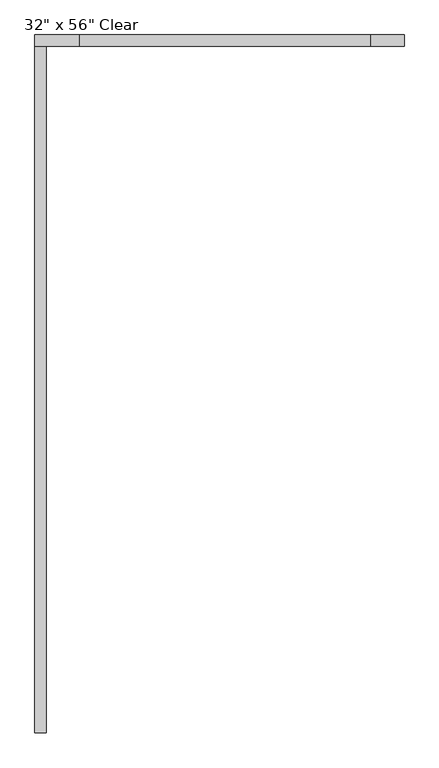
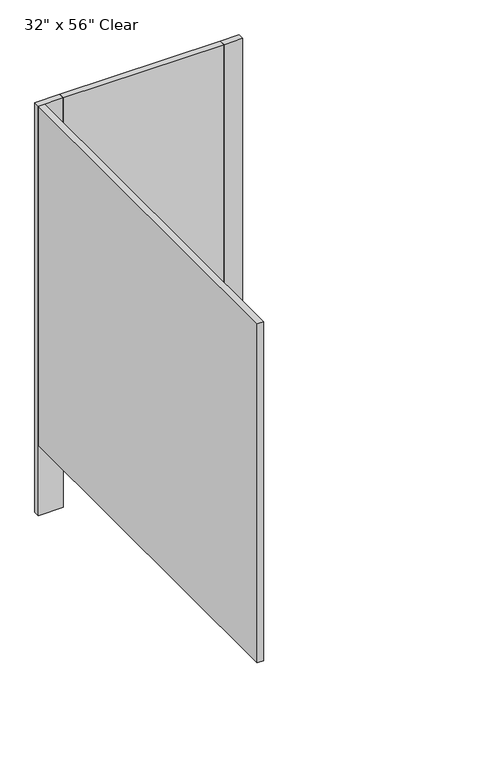
"""IFC4 building model written with IfcOpenShell, lengths in millimetres: proxy geometry."""

from ifc_helpers import new_model, si_unit, frame, origin, origin_with_axes, place, context, project, spatial, polyline, outline, extrude, source, transform, mapped, element, save


def proxy_86d28e76(model_context):
    return source(origin(), model_context, "Body", "SweptSolid", [
        extrude(outline(polyline([(735.1031538, 1646.2375), (735.1031538, 1620.8375), (74.7031538, 1620.8375), (74.7031538, 1646.2375), (735.1031538, 1646.2375)])), frame((0.0, 0.0, 304.8), z_axis=(0.0, 0.0, 1.0), x_axis=(1.0, 0.0, 0.0)), (0.0, 0.0, 1.0), 1473.2),
        extrude(outline(polyline([(74.7031538, 1646.2375), (74.7031538, 1620.8375), (-26.8968462, 1620.8375), (-26.8968462, 1646.2375), (74.7031538, 1646.2375)])), origin_with_axes(), (0.0, 0.0, 1.0), 1778.0),
        extrude(outline(polyline([(811.3031538, 1646.2375), (811.3031538, 1620.8375), (735.1031538, 1620.8375), (735.1031538, 1646.2375), (811.3031538, 1646.2375)])), origin_with_axes(), (0.0, 0.0, 1.0), 1778.0),
        extrude(outline(polyline([(-26.8968462, 1620.8375), (-1.4968462, 1620.8375), (-1.4968462, 63.5), (-26.8968462, 63.5), (-26.8968462, 1620.8375)])), frame((0.0, 0.0, 304.8), z_axis=(0.0, 0.0, 1.0), x_axis=(1.0, 0.0, 0.0)), (0.0, 0.0, 1.0), 1473.2),
    ])


if __name__ == "__main__":
    model = new_model("IFC4")
    model_context = context("Model", 3, world=origin())
    ifc_project = project(units=[si_unit("LENGTHUNIT", "METRE", prefix="MILLI")], contexts=[model_context])
    site = spatial("IfcSite", under=ifc_project)
    building = spatial("IfcBuilding", under=site)
    placement = place(None, origin())
    proxy_shape = proxy_86d28e76(model_context)
    element("IfcBuildingElementProxy", 1, Name="Toilet Stall-3D w Toilet : 32\" x 56\" Clear", ObjectType="Toilet Stall-3D w Toilet : 32\" x 56\" Clear", at=placement, inside=building, context=model_context, shape_type="MappedRepresentation", body=[
        mapped(proxy_shape, transform((0.0, 0.0, 0.0), x_axis=(1.0, 0.0, 0.0), y_axis=(0.0, 1.0, 0.0), z_axis=(0.0, 0.0, 1.0))),
    ])
    save(model, "model.ifc")

# Revit data of these elements
# Type "Toilet Stall-3D w Toilet : 32\" x 56\" Clear"
#   Assembly Code = "C1030100"
#   Door Width = 2' - 2"
#   Length = 4' - 8"
#   Width = 2' - 8"
#   Toilet Partition Material = Toilet Partition
#   Default Elevation = 0
# Element 1 (IfcBuildingElementProxy, "Toilet Stall-3D w Toilet : 32\" x 56\" Clear")
#   Materials on its faces: "Toilet Partition"
# Materials
#   "Toilet Partition": class "Unassigned", colour RGB 0 181 188, transparency 0
